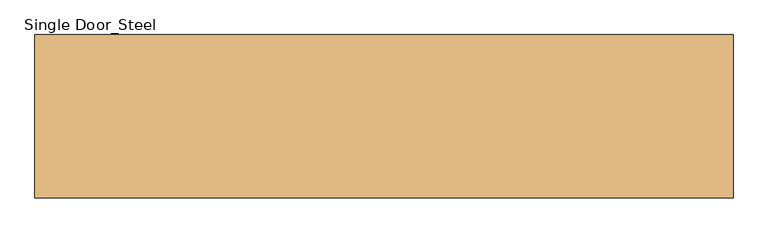
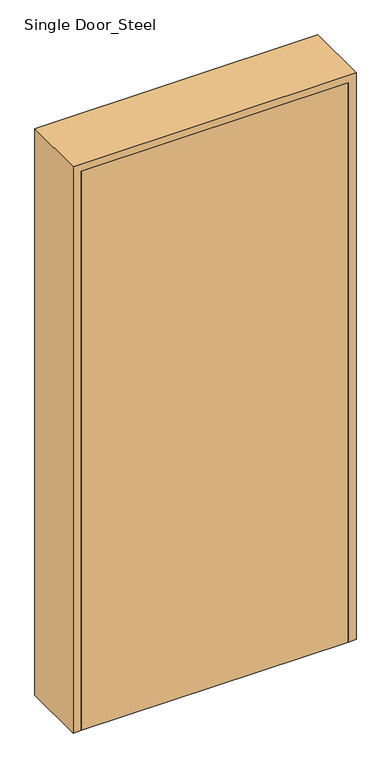
"""IFC4 building model written with IfcOpenShell, lengths in millimetres: door geometry, Single Door_Steel : H_DR_AR B12_Door_Single_W1100xH2280_FR 1.0H_FSD-2."""

from ifc_helpers import new_model, si_unit, origin, origin_with_axes, place, context, project, spatial, polyline, outline, extrude, faceted_brep, source, transform, mapped, element, save


def single_door_steel_5f783c26(model_context):
    return source(origin(), model_context, "Body", "SolidModel", [
        extrude(outline(polyline([(505.0, -125.0), (-505.0, -125.0), (-505.0, -85.0), (505.0, -85.0), (505.0, -125.0)])), origin_with_axes(), (0.0, 0.0, 1.0), 2235.0),
        faceted_brep([(505.0, -125.0, 0.0), (505.0, -85.0, 0.0), (485.0, -85.0, 0.0), (485.0, 85.0, 0.0), (505.0, 85.0, 0.0), (505.0, 125.0, 0.0), (535.0, 125.0, 0.0), (535.0, -125.0, 0.0), (535.0, -125.0, 2265.0), (-535.0, -125.0, 2265.0), (-535.0, -125.0, 0.0), (-505.0, -125.0, 0.0), (-505.0, -125.0, 2235.0), (505.0, -125.0, 2235.0), (535.0, 125.0, 2265.0), (505.0, 125.0, 2235.0), (-505.0, 125.0, 2235.0), (-505.0, 125.0, 0.0), (-535.0, 125.0, 0.0), (-535.0, 125.0, 2265.0), (505.0, 85.0, 2235.0), (485.0, 85.0, 2215.0), (-485.0, 85.0, 2215.0), (-485.0, 85.0, 0.0), (-505.0, 85.0, 0.0), (-505.0, 85.0, 2235.0), (485.0, -85.0, 2215.0), (505.0, -85.0, 2235.0), (-505.0, -85.0, 2235.0), (-505.0, -85.0, 0.0), (-485.0, -85.0, 0.0), (-485.0, -85.0, 2215.0)], [[[0, 1, 2, 3, 4, 5, 6, 7]], [[7, 8, 9, 10, 11, 12, 13, 0]], [[6, 14, 8, 7]], [[5, 15, 16, 17, 18, 19, 14, 6]], [[4, 20, 15, 5]], [[3, 21, 22, 23, 24, 25, 20, 4]], [[2, 26, 21, 3]], [[1, 27, 28, 29, 30, 31, 26, 2]], [[0, 13, 27, 1]], [[12, 11, 29, 28]], [[11, 10, 18, 17, 24, 23, 30, 29]], [[19, 18, 10, 9]], [[25, 24, 17, 16]], [[31, 30, 23, 22]], [[14, 19, 9, 8]], [[20, 25, 16, 15]], [[26, 31, 22, 21]], [[13, 12, 28, 27]]]),
    ])


if __name__ == "__main__":
    model = new_model("IFC4")
    model_context = context("Model", 3, world=origin())
    ifc_project = project(units=[si_unit("LENGTHUNIT", "METRE", prefix="MILLI")], contexts=[model_context])
    site = spatial("IfcSite", under=ifc_project)
    building = spatial("IfcBuilding", under=site)
    placement = place(None, origin())
    single_door_steel_shape = single_door_steel_5f783c26(model_context)
    element("IfcDoor", 1, ObjectType="Single Door_Steel : H_DR_AR B12_Door_Single_W1100xH2280_FR 1.0H_FSD-2", at=placement, inside=building, context=model_context, shape_type="MappedRepresentation", body=[
        mapped(single_door_steel_shape, transform((0.0, 0.0, 0.0), x_axis=(1.0, 0.0, 0.0), y_axis=(0.0, 1.0, 0.0), z_axis=(0.0, 0.0, 1.0))),
    ])
    save(model, "model.ifc")

# Revit data of these elements
# Type "Single Door_Steel : H_DR_AR B12_Door_Single_W1100xH2280_FR 1.0H_FSD-2"
#   Type Mark = "442"
#   Analytic Construction = "<None>"
#   프레임 투영 외부. = 25 mm
#   프레임 투영 내부. = 25 mm
#   프레임 폭 = 75 mm
#   Height = 2280 mm
#   Width = 1100 mm
#   Define Thermal Properties by = 1
#   문 패널 = none
#   문 프레임 = none
#   Function = (empty or 0)
#   Wall Closure = (empty or 0)
